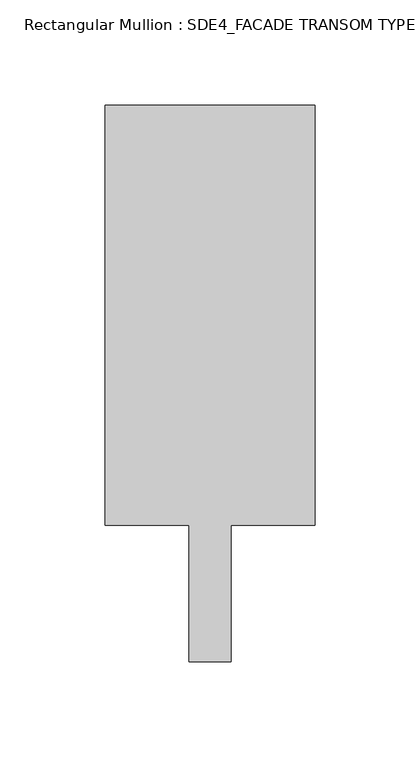
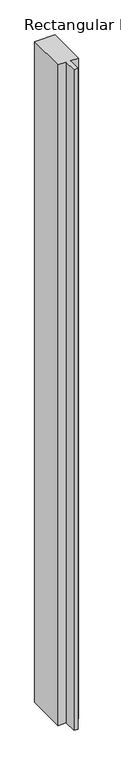
"""IFC4 building model written with IfcOpenShell, lengths in millimetres: member geometry, Rectangular Mullion : SDE4_FACADE TRANSOM TYPE 2."""

from ifc_helpers import new_model, si_unit, frame, origin, place, context, project, spatial, polyline, outline, extrude, source, transform, mapped, element, save


def rectangular_mullion_sde4_facade_transom_type_2_d4ced0e5(model_context):
    return source(origin(), model_context, "Body", "SweptSolid", [
        extrude(outline(polyline([(50.0, 132.5), (50.0, -67.5), (10.0, -67.5), (10.0, -132.5), (-10.0, -132.5), (-10.0, -67.5), (-50.0, -67.5), (-50.0, 132.5), (50.0, 132.5)])), frame((0.0, 0.0, -3439.0), z_axis=(0.0, 0.0, 1.0), x_axis=(1.0, 0.0, 0.0)), (0.0, 0.0, 1.0), 3439.0),
    ])


if __name__ == "__main__":
    model = new_model("IFC4")
    model_context = context("Model", 3, world=origin())
    ifc_project = project(units=[si_unit("LENGTHUNIT", "METRE", prefix="MILLI")], contexts=[model_context])
    site = spatial("IfcSite", under=ifc_project)
    building = spatial("IfcBuilding", under=site)
    placement = place(None, origin())
    rectangular_mullion_sde4_facade_transom_type_2_shape = rectangular_mullion_sde4_facade_transom_type_2_d4ced0e5(model_context)
    element("IfcMember", 1, ObjectType="Rectangular Mullion : SDE4_FACADE TRANSOM TYPE 2", at=placement, inside=building, context=model_context, shape_type="MappedRepresentation", body=[
        mapped(rectangular_mullion_sde4_facade_transom_type_2_shape, transform((0.0, 0.0, 0.0), x_axis=(1.0, 0.0, 0.0), y_axis=(0.0, 1.0, 0.0), z_axis=(0.0, 0.0, 1.0))),
    ])
    save(model, "model.ifc")

# Revit data of these elements
# Type "Rectangular Mullion : SDE4_FACADE TRANSOM TYPE 2"
#   built-in parameter 1007322 = 0.869423 (stored number, unit not read)
#   built-in parameter 1007321 = 0.164042 (stored number, unit not read)
#   built-in parameter 1007320 = 0.164042 (stored number, unit not read)
